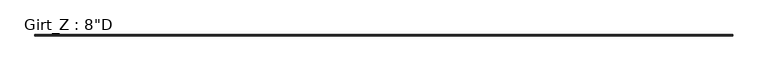
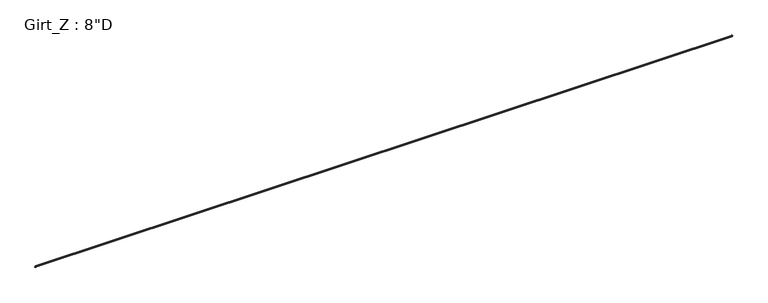
"""IFC4 building model written with IfcOpenShell, lengths in millimetres: beam geometry."""

from ifc_helpers import new_model, si_unit, point, frame, frame_2d, origin, place, context, project, spatial, polyline, circle_curve, trimmed, segment, composite_curve, outline, extrude, source, transform, mapped, element, save


def beam_1069c96b(model_context):
    return source(origin(), model_context, "Body", "SweptSolid", [
        extrude(outline(composite_curve([segment(polyline([(-63.5, 101.6), (-3.3734375, 101.6)]), True, "CONTINUOUS"), segment(trimmed(circle_curve(frame_2d((-3.3734375, 96.8375)), 4.7625), [point((-3.3734375, 101.6))], [point((1.3890625, 96.8375))], False, "CARTESIAN"), True, "CONTINUOUS"), segment(polyline([(1.3890625, 96.8375), (1.3890625, -96.8389339)]), True, "CONTINUOUS"), segment(trimmed(circle_curve(frame_2d((3.3748024, -96.8389339)), 1.9857399), [point((1.3890625, -96.8389339))], [point((3.2694106, -98.821875))], True, "CARTESIAN"), True, "CONTINUOUS"), segment(polyline([(3.2694106, -98.821875), (62.204539, -98.821875), (73.6169367, -85.221109), (75.745104, -87.0068534), (63.5, -101.6), (3.3734375, -101.6)]), True, "CONTINUOUS"), segment(trimmed(circle_curve(frame_2d((3.3734375, -96.8375)), 4.7625), [point((3.3734375, -101.6))], [point((-1.3890625, -96.8375))], False, "CARTESIAN"), True, "CONTINUOUS"), segment(polyline([(-1.3890625, -96.8375), (-1.3890625, 96.8381931)]), True, "CONTINUOUS"), segment(trimmed(circle_curve(frame_2d((-3.3741066, 96.8381931)), 1.9850441), [point((-1.3890625, 96.8381931))], [point((-3.3005807, 98.821875))], True, "CARTESIAN"), True, "CONTINUOUS"), segment(polyline([(-3.3005807, 98.821875), (-62.204539, 98.821875), (-73.6169367, 85.221109), (-75.745104, 87.0068534), (-63.5, 101.6)]), True, "CONTINUOUS")], self_intersect=False)), frame((-40602.569726, 0.0, 0.0), z_axis=(1.0, 0.0, 0.0), x_axis=(0.0, 1.0, 0.0)), (0.0, 0.0, 1.0), 81057.5019525),
    ])


if __name__ == "__main__":
    model = new_model("IFC4")
    model_context = context("Model", 3, world=origin())
    ifc_project = project(units=[si_unit("LENGTHUNIT", "METRE", prefix="MILLI")], contexts=[model_context])
    site = spatial("IfcSite", under=ifc_project)
    building = spatial("IfcBuilding", under=site)
    placement = place(None, origin())
    beam_shape = beam_1069c96b(model_context)
    element("IfcBeam", 1, ObjectType="Girt_Z : 8\"D", at=placement, inside=building, context=model_context, shape_type="MappedRepresentation", body=[
        mapped(beam_shape, transform((0.0, 0.0, 0.0), x_axis=(1.0, 0.0, 0.0), y_axis=(0.0, 1.0, 0.0), z_axis=(0.0, 0.0, 1.0))),
    ])
    save(model, "model.ifc")

# Revit data of these elements
# Type "Girt_Z : 8\"D"
#   Web_Thickness = 0' - 0 7/64"
#   Length [instance default] = 10' - 0"
#   Leg_1 = 0' - 2 1/2"
#   Height = 0' - 8"
#   Structural Material [instance default] = none
# Element 1 (IfcBeam, "Girt_Z : 8\"D")
#   Structural Material = Steel
#   Materials on its faces: "Steel"
# Materials
#   "Steel": class "Metal", colour RGB 118 118 114, transparency 0, Description = "Steel, mill finish", Cost = 0
